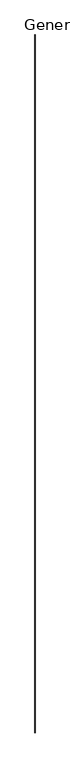
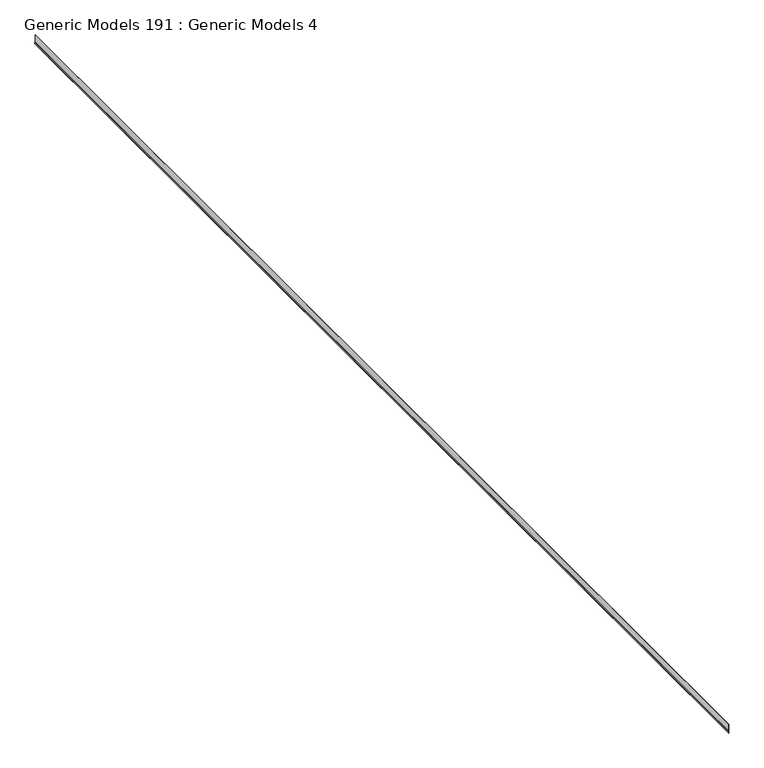
"""IFC4 building model written with IfcOpenShell, lengths in millimetres: proxy geometry, Generic Models 191 : Generic Models 4."""

from ifc_helpers import new_model, si_unit, frame, origin, place, context, project, spatial, polyline, outline, extrude, source, transform, mapped, element, save


def generic_models_191_generic_models_4_13d6aea7(model_context):
    return source(origin(), model_context, "Body", "SweptSolid", [
        extrude(outline(polyline([(129257.5595277, -5331.7923796), (129376.8012418, -5331.7923796), (129376.8012418, -5332.5861296), (129257.6994872, -5332.5861296), (129246.605741, -5336.623923), (129231.5519784, -5336.623923), (129231.5519784, -5335.830173), (129246.4657814, -5335.830173), (129257.5595277, -5331.7923796)])), frame((0.0, -6864.9230338, 0.0), z_axis=(0.0, 1.0, 0.0), x_axis=(0.0, 0.0, 1.0)), (0.0, 0.0, 1.0), 18643.6),
    ])


if __name__ == "__main__":
    model = new_model("IFC4")
    model_context = context("Model", 3, world=origin())
    ifc_project = project(units=[si_unit("LENGTHUNIT", "METRE", prefix="MILLI")], contexts=[model_context])
    site = spatial("IfcSite", under=ifc_project)
    building = spatial("IfcBuilding", under=site)
    placement = place(None, origin())
    generic_models_191_generic_models_4_shape = generic_models_191_generic_models_4_13d6aea7(model_context)
    element("IfcBuildingElementProxy", 1, Name="Generic Models 191 : Generic Models 4", ObjectType="Generic Models 191 : Generic Models 4", at=placement, inside=building, context=model_context, shape_type="MappedRepresentation", body=[
        mapped(generic_models_191_generic_models_4_shape, transform((0.0, 0.0, 0.0), x_axis=(1.0, 0.0, 0.0), y_axis=(0.0, 1.0, 0.0), z_axis=(0.0, 0.0, 1.0))),
    ])
    save(model, "model.ifc")

# Revit data of these elements
# Element 1 (IfcBuildingElementProxy, "Generic Models 191 : Generic Models 4")
#   Materials on its faces: "_(2) LAYERS NO. 30 ASTM D226 ASPHALT SATURATED ORGANIC FELT"
# Materials
#   "_(2) LAYERS NO. 30 ASTM D226 ASPHALT SATURATED ORGANIC FELT": class "Generic", colour RGB 67 154 161, transparency 0, Cost = 0
